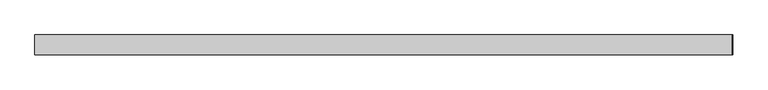
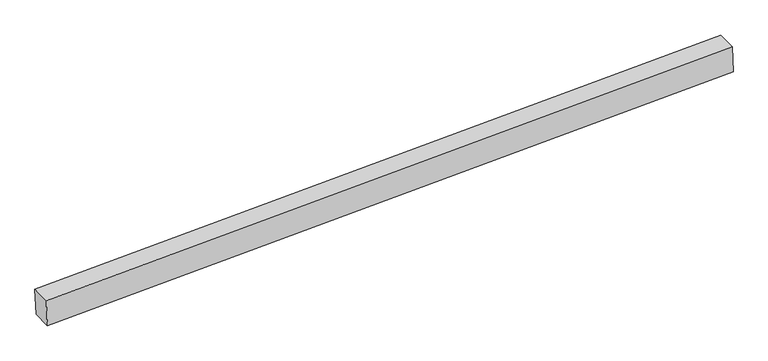
"""IFC4 building model written with IfcOpenShell, lengths in millimetres: proxy geometry, Generic Models 7:Generic Models 1:8:Generic Models 1:8 : Generic Models 7:Generic Models 1:337419:34 : Generic Models 7:Generic Models 1:8:Generic Models 1:8 : Generic Models 7:Generic Models 1:337419:315935."""

from ifc_helpers import new_model, si_unit, frame, origin, place, context, project, spatial, polyline, outline, extrude, source, transform, mapped, element, save


def generic_models_97c9fb10(model_context):
    return source(origin(), model_context, "Body", "SweptSolid", [
        extrude(outline(polyline([(3818.9012888, 558136.9256261), (3628.5664384, 558144.8562449), (3831.5897382, 563017.4154421), (4021.9397427, 563009.8485204), (3818.9012888, 558136.9256261)])), frame((0.0, -578791.1413841, 0.0), z_axis=(0.0, 1.0, 0.0), x_axis=(0.0, 0.0, 1.0)), (0.0, 0.0, 1.0), 139.7),
    ])


if __name__ == "__main__":
    model = new_model("IFC4")
    model_context = context("Model", 3, world=origin())
    ifc_project = project(units=[si_unit("LENGTHUNIT", "METRE", prefix="MILLI")], contexts=[model_context])
    site = spatial("IfcSite", under=ifc_project)
    building = spatial("IfcBuilding", under=site)
    placement = place(None, origin())
    generic_models_shape = generic_models_97c9fb10(model_context)
    element("IfcBuildingElementProxy", 1, Name="Generic Models 7:Generic Models 1:8:Generic Models 1:8 : Generic Models 7:Generic Models 1:337419:34 : Generic Models 7:Generic Models 1:8:Generic Models 1:8 : Generic Models 7:Generic Models 1:337419:315935", ObjectType="Generic Models 7:Generic Models 1:8:Generic Models 1:8 : Generic Models 7:Generic Models 1:337419:34 : Generic Models 7:Generic Models 1:8:Generic Models 1:8 : Generic Models 7:Generic Models 1:337419:315935", at=placement, inside=building, context=model_context, shape_type="MappedRepresentation", body=[
        mapped(generic_models_shape, transform((0.0, 0.0, 0.0), x_axis=(1.0, 0.0, 0.0), y_axis=(0.0, 1.0, 0.0), z_axis=(0.0, 0.0, 1.0))),
    ])
    save(model, "model.ifc")

# Revit data of these elements
# Type "Generic Models 7:Generic Models 1:8:Generic Models 1:8 : Generic Models 7:Generic Models 1:337419:34 : Generic Models 7:Generic Models 1:8:Generic Models 1:8 : Generic Models 7:Generic Models 1:337419:315935"
#   NameOverride = "Generic Models 7:Generic Models 1:8:Generic Models 1:8 : Generic Models 7:Generic Models 1:337419:315935"
#   ObjectTypeOverride = "Generic Models 1:8 : Generic Models 7:Generic Models 1:337419"
#   Reference = "Generic Models 1"
#   Tag = "315935"
# Element 1 (IfcBuildingElementProxy, "Generic Models 7:Generic Models 1:8:Generic Models 1:8 : Generic Models 7:Generic Models 1:337419:34 : Generic Models 7:Generic Models 1:8:Generic Models 1:8 : Generic Models 7:Generic Models 1:337419:315935")
#   Materials on its faces: "5 1/2\" X 7 1/2\" EXTERIOR GRADE GLULAM BEAMS"
# Materials
#   "5 1/2\" X 7 1/2\" EXTERIOR GRADE GLULAM BEAMS": class "Wood", colour RGB 183 134 68, transparency 0, Keynote = "M06181300.01", Description = "Pinus Echinata", Cost = 0
